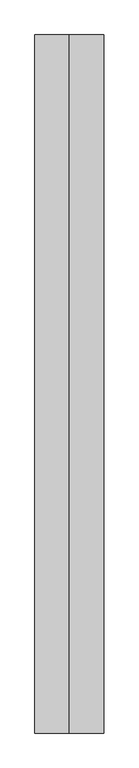
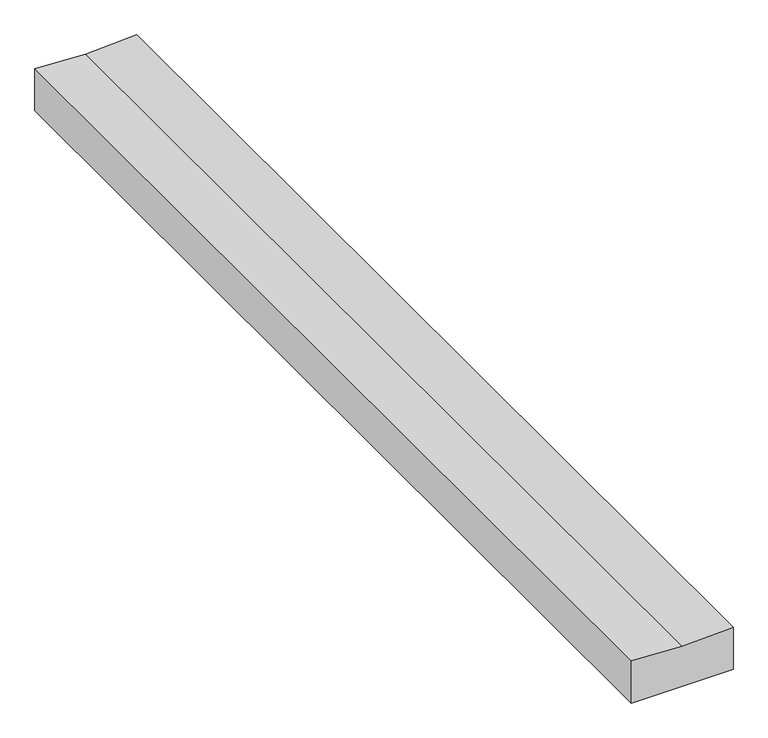
"""IFC4 building model written with IfcOpenShell, lengths in millimetres: proxy geometry, FIRESTONE INSULATION002 : FIRESTONE INSULATION002."""

from ifc_helpers import new_model, si_unit, frame, origin, place, context, project, spatial, polyline, outline, extrude, source, transform, mapped, element, save


def generic_models_8e6e040b(model_context):
    return source(origin(), model_context, "Body", "SweptSolid", [
        extrude(outline(polyline([(40131.746, -4797.9038825), (40131.746, -4601.0538825), (40218.4000089, -4601.0538825), (40213.3984375, -4699.8063764), (40218.4000089, -4797.9038825), (40131.746, -4797.9038825)])), frame((0.0, -1052.6406573, 0.0), z_axis=(0.0, 1.0, 0.0), x_axis=(0.0, 0.0, 1.0)), (0.0, 0.0, 1.0), 2000.0),
    ])


if __name__ == "__main__":
    model = new_model("IFC4")
    model_context = context("Model", 3, world=origin())
    ifc_project = project(units=[si_unit("LENGTHUNIT", "METRE", prefix="MILLI")], contexts=[model_context])
    site = spatial("IfcSite", under=ifc_project)
    building = spatial("IfcBuilding", under=site)
    placement = place(None, origin())
    generic_models_shape = generic_models_8e6e040b(model_context)
    element("IfcBuildingElementProxy", 1, Name="FIRESTONE INSULATION002 : FIRESTONE INSULATION002", ObjectType="FIRESTONE INSULATION002 : FIRESTONE INSULATION002", at=placement, inside=building, context=model_context, shape_type="MappedRepresentation", body=[
        mapped(generic_models_shape, transform((0.0, 0.0, 0.0), x_axis=(1.0, 0.0, 0.0), y_axis=(0.0, 1.0, 0.0), z_axis=(0.0, 0.0, 1.0))),
    ])
    save(model, "model.ifc")

# Revit data of these elements
# Type "FIRESTONE INSULATION002 : FIRESTONE INSULATION002"
#   NameOverride = "FIRESTONE INSULATION002"
# Element 1 (IfcBuildingElementProxy, "FIRESTONE INSULATION002 : FIRESTONE INSULATION002")
#   Materials on its faces: "TAPERED 2X SLEEPERS - SLOPED TO DRAIN"
# Materials
#   "TAPERED 2X SLEEPERS - SLOPED TO DRAIN": class "Unassigned", colour RGB 234 198 178, transparency 0
